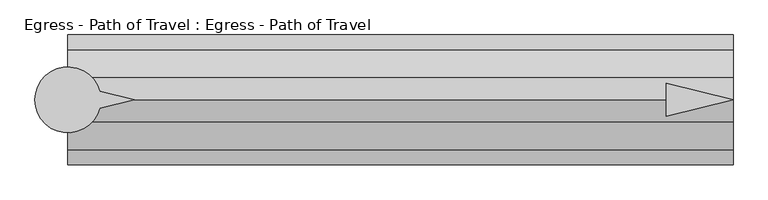
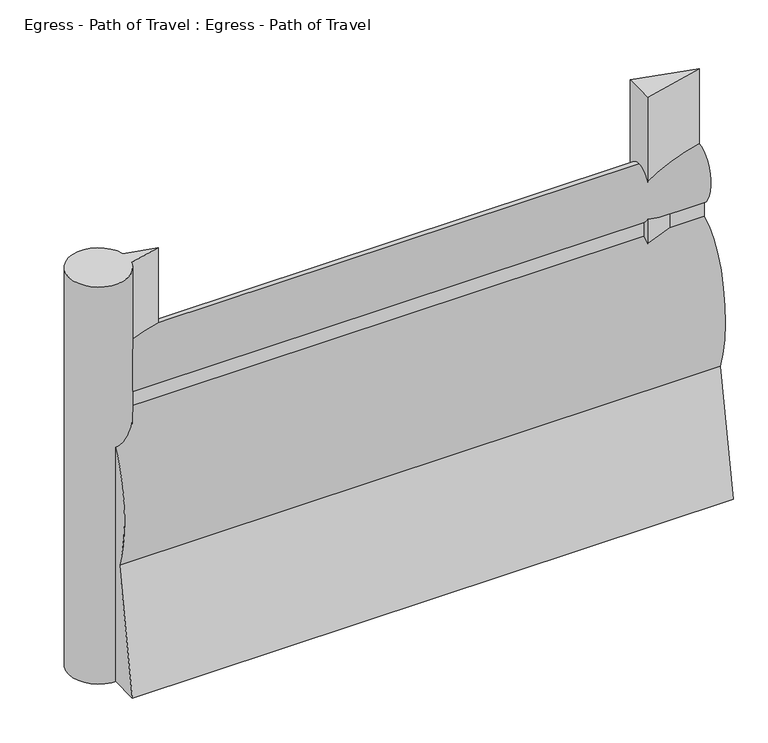
"""IFC4 building model written with IfcOpenShell, lengths in millimetres: proxy geometry, Egress - Path of Travel : Egress - Path of Travel."""

from ifc_helpers import new_model, si_unit, point, frame, frame_2d, origin, origin_with_axes, place, context, project, spatial, polyline, circle_curve, ellipse_curve, trimmed, segment, composite_curve, outline, extrude, source, transform, mapped, element, save
from ifc_brep_helpers import plane_surface, extruded_surface, advanced_brep


def egress_path_of_travel_egress_path_of_travel_d5dfa4f0(model_context):
    return source(origin(), model_context, "Body", "SolidModel", [
        advanced_brep(
        [(227.5554837, 0.0, 1727.2), (227.5554837, 42.9018657, 1436.6534209), (227.5554837, 42.9018657, 1363.4763406), (227.5554837, 184.1186263, 643.4144547), (227.5554837, 297.5699544, 0.0), (227.5554837, 145.6574193, 0.0), (227.5554837, 0.0, 584.2), (227.5554837, -145.6574193, 0.0), (227.5554837, -297.5699544, 0.0), (227.5554837, -184.1186263, 643.4144547), (227.5554837, -42.9018657, 1363.4763406), (227.5554837, -42.9018657, 1436.6534209), (3275.5554837, 0.0, 1727.2), (3275.5554837, -42.9018657, 1436.6534209), (3275.5554837, -42.9018657, 1363.4763406), (3275.5554837, -184.1186263, 643.4144547), (3275.5554837, -297.5699544, 0.0), (3275.5554837, -145.6574193, 0.0), (3275.5554837, 0.0, 584.2), (3275.5554837, 145.6574193, 0.0), (3275.5554837, 297.5699544, 0.0), (3275.5554837, 184.1186263, 643.4144547), (3275.5554837, 42.9018657, 1363.4763406), (3275.5554837, 42.9018657, 1436.6534209)],
        [
            (0, 1, ellipse_curve(frame((227.5554837, 0.0, 1574.8), z_axis=(-1.0, 0.0, 0.0), x_axis=(0.0, 0.0, 1.0)), 152.4, 101.6)),
            (1, 2),
            (2, 3, ellipse_curve(frame((227.5554837, 0.0, 914.4), z_axis=(-1.0, 0.0, 0.0), x_axis=(0.0, 0.0, -1.0)), 457.2, 228.6)),
            (3, 4),
            (4, 5),
            (5, 6),
            (6, 7),
            (7, 8),
            (8, 9),
            (9, 10, ellipse_curve(frame((227.5554837, 0.0, 914.4), z_axis=(-1.0, 0.0, 0.0), x_axis=(0.0, 0.0, -1.0)), 457.2, 228.6)),
            (10, 11),
            (11, 0, ellipse_curve(frame((227.5554837, 0.0, 1574.8), z_axis=(-1.0, 0.0, 0.0), x_axis=(0.0, 0.0, 1.0)), 152.4, 101.6)),
            (12, 13, ellipse_curve(frame((3275.5554837, 0.0, 1574.8), z_axis=(1.0, 0.0, 0.0), x_axis=(0.0, 0.0, 1.0)), 152.4, 101.6)),
            (13, 14),
            (14, 15, ellipse_curve(frame((3275.5554837, 0.0, 914.4), z_axis=(1.0, 0.0, 0.0), x_axis=(0.0, 0.0, -1.0)), 457.2, 228.6)),
            (15, 16),
            (16, 17),
            (17, 18),
            (18, 19),
            (19, 20),
            (20, 21),
            (21, 22, ellipse_curve(frame((3275.5554837, 0.0, 914.4), z_axis=(1.0, 0.0, 0.0), x_axis=(0.0, 0.0, -1.0)), 457.2, 228.6)),
            (22, 23),
            (23, 12, ellipse_curve(frame((3275.5554837, 0.0, 1574.8), z_axis=(1.0, 0.0, 0.0), x_axis=(0.0, 0.0, 1.0)), 152.4, 101.6)),
            (0, 12),
            (23, 1),
            (22, 2),
            (21, 3),
            (20, 4),
            (19, 5),
            (18, 6),
            (17, 7),
            (16, 8),
            (15, 9),
            (14, 10),
            (13, 11),
        ],
        [
            plane_surface(frame((227.5554837, 0.0, 0.0), z_axis=(-1.0, 0.0, 0.0), x_axis=(0.0, 0.0, 1.0))),
            plane_surface(frame((3275.5554837, 0.0, 0.0), z_axis=(1.0, 0.0, 0.0), x_axis=(0.0, 0.0, 1.0))),
            extruded_surface(trimmed(ellipse_curve(frame((3275.5554837, 0.0, 1574.8), z_axis=(-1.0, 0.0, 0.0), x_axis=(0.0, 0.0, 1.0)), 152.4, 101.6), [point((3275.5554837, 0.0, 1727.2))], [point((3275.5554837, 42.9018657, 1436.6534209))], True, "CARTESIAN"), (-3048.0, 0.0, 0.0), 3048.0),
            plane_surface(frame((227.5554837, 42.9018657, 1436.6534209), z_axis=(0.0, 1.0, 0.0), x_axis=(1.0, 0.0, 0.0))),
            extruded_surface(trimmed(ellipse_curve(frame((3275.5554837, 0.0, 914.4), z_axis=(-1.0, 0.0, 0.0), x_axis=(0.0, 0.0, -1.0)), 457.2, 228.6), [point((3275.5554837, 42.9018657, 1363.4763406))], [point((3275.5554837, 184.1186263, 643.4144547))], True, "CARTESIAN"), (-3048.0, 0.0, 0.0), 3048.0),
            plane_surface(frame((227.5554837, 184.1186263, 643.4144547), z_axis=(0.0, 0.9848077530122078, 0.1736481776669322), x_axis=(1.0, 0.0, 0.0))),
            plane_surface(frame((227.5554837, 297.5699544, 0.0), z_axis=(0.0, 0.0, -1.0), x_axis=(1.0, 0.0, 0.0))),
            plane_surface(frame((227.5554837, 145.6574193, 0.0), z_axis=(0.0, -0.9702957262760199, -0.2419218955995739), x_axis=(1.0, 0.0, 0.0))),
            plane_surface(frame((227.5554837, 0.0, 584.2), z_axis=(0.0, 0.9702957262759961, -0.24192189559966923), x_axis=(1.0, 0.0, 0.0))),
            plane_surface(frame((227.5554837, -145.6574193, 0.0), z_axis=(0.0, 0.0, -1.0), x_axis=(1.0, 0.0, 0.0))),
            plane_surface(frame((227.5554837, -297.5699544, 0.0), z_axis=(0.0, -0.984807753012208, 0.17364817766693066), x_axis=(1.0, 0.0, 0.0))),
            extruded_surface(trimmed(ellipse_curve(frame((3275.5554837, 0.0, 914.4), z_axis=(-1.0, 0.0, 0.0), x_axis=(0.0, 0.0, -1.0)), 457.2, 228.6), [point((3275.5554837, -184.1186263, 643.4144547))], [point((3275.5554837, -42.9018657, 1363.4763406))], True, "CARTESIAN"), (-3048.0, 0.0, 0.0), 3048.0),
            plane_surface(frame((227.5554837, -42.9018657, 1363.4763406), z_axis=(0.0, -1.0, 0.0), x_axis=(1.0, 0.0, 0.0))),
            extruded_surface(trimmed(ellipse_curve(frame((3275.5554837, 0.0, 1574.8), z_axis=(-1.0, 0.0, 0.0), x_axis=(0.0, 0.0, 1.0)), 152.4, 101.6), [point((3275.5554837, -42.9018657, 1436.6534209))], [point((3275.5554837, 0.0, 1727.2))], True, "CARTESIAN"), (-3048.0, 0.0, 0.0), 3048.0),
        ],
        [
            (0, [[1, 2, 3, 4, 5, 6, 7, 8, 9, 10, 11, 12]]),
            (1, [[13, 14, 15, 16, 17, 18, 19, 20, 21, 22, 23, 24]]),
            (2, [[-1, 25, -24, 26]]),
            (3, [[-2, -26, -23, 27]]),
            (4, [[-3, -27, -22, 28]]),
            (5, [[-4, -28, -21, 29]]),
            (6, [[-5, -29, -20, 30]]),
            (7, [[-6, -30, -19, 31]]),
            (8, [[-7, -31, -18, 32]]),
            (9, [[-8, -32, -17, 33]]),
            (10, [[-9, -33, -16, 34]]),
            (11, [[-10, -34, -15, 35]]),
            (12, [[-11, -35, -14, 36]]),
            (13, [[-12, -36, -13, -25]]),
        ],
    ),
        extrude(outline(polyline([(2969.5503371, 76.2006338), (3275.5554837, 0.0), (2969.5503371, -76.2006338), (2969.5503371, 76.2006338)])), origin_with_axes(), (0.0, 0.0, 1.0), 2129.5973753),
        extrude(outline(composite_curve([segment(polyline([(372.7837828, 39.4440225), (531.182385, 0.0), (372.7837828, -39.4440225)]), True, "CONTINUOUS"), segment(trimmed(circle_curve(frame_2d((227.2200886, 0.0)), 150.8131956), [point((372.7837828, -39.4440225))], [point((372.7837828, 39.4440225))], False, "CARTESIAN"), True, "CONTINUOUS")], self_intersect=False)), origin_with_axes(), (0.0, 0.0, 1.0), 2129.5973753),
    ])


if __name__ == "__main__":
    model = new_model("IFC4")
    model_context = context("Model", 3, world=origin())
    ifc_project = project(units=[si_unit("LENGTHUNIT", "METRE", prefix="MILLI")], contexts=[model_context])
    site = spatial("IfcSite", under=ifc_project)
    building = spatial("IfcBuilding", under=site)
    placement = place(None, origin())
    egress_path_of_travel_egress_path_of_travel_shape = egress_path_of_travel_egress_path_of_travel_d5dfa4f0(model_context)
    element("IfcBuildingElementProxy", 1, Name="Egress - Path of Travel : Egress - Path of Travel", ObjectType="Egress - Path of Travel : Egress - Path of Travel", at=placement, inside=building, context=model_context, shape_type="MappedRepresentation", body=[
        mapped(egress_path_of_travel_egress_path_of_travel_shape, transform((0.0, 0.0, 0.0), x_axis=(1.0, 0.0, 0.0), y_axis=(0.0, 1.0, 0.0), z_axis=(0.0, 0.0, 1.0))),
    ])
    save(model, "model.ifc")

# Revit data of these elements
# Type "Egress - Path of Travel : Egress - Path of Travel"
#   Path of Egress [instance default] = 4' - 0"
#   built-in parameter 1001306 [instance default] = 4 (stored number, unit not read)
#   Dot at Start = no
#   Arrow in Middle = yes
#   Arrow at End = no
#   Egress Path = none
# Element 1 (IfcBuildingElementProxy, "Egress - Path of Travel : Egress - Path of Travel")
#   Path of Egress = 10' - 0"
#   built-in parameter 1001306 = 10 (stored number, unit not read)
